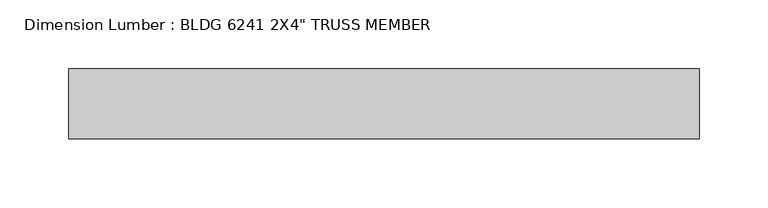
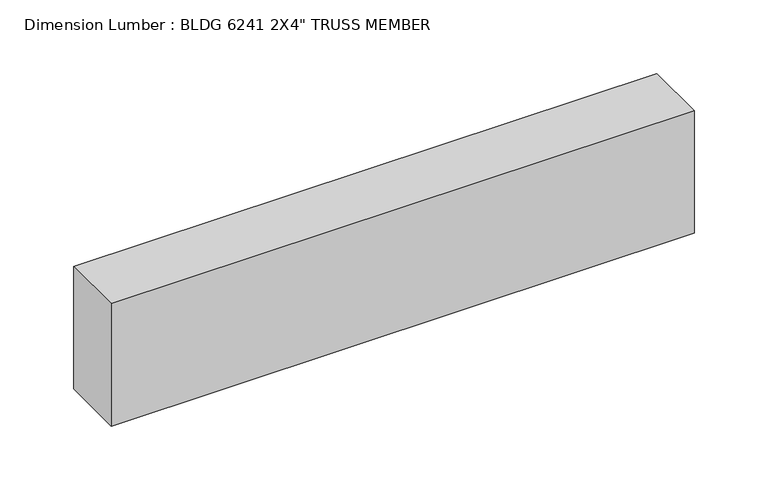
"""IFC4 building model written with IfcOpenShell, lengths in millimetres: beam geometry."""

from ifc_helpers import new_model, si_unit, frame, origin, place, context, project, spatial, polyline, outline, extrude, source, transform, mapped, element, save


def beam_154fe962(model_context):
    return source(origin(), model_context, "Body", "SweptSolid", [
        extrude(outline(polyline([(228.5999994, 25.4), (228.5999994, -25.4), (-228.6, -25.4), (-228.6, 25.4), (228.5999994, 25.4)])), frame((0.0, 0.0, -50.8), z_axis=(0.0, 0.0, 1.0), x_axis=(1.0, 0.0, 0.0)), (0.0, 0.0, 1.0), 101.6),
    ])


if __name__ == "__main__":
    model = new_model("IFC4")
    model_context = context("Model", 3, world=origin())
    ifc_project = project(units=[si_unit("LENGTHUNIT", "METRE", prefix="MILLI")], contexts=[model_context])
    site = spatial("IfcSite", under=ifc_project)
    building = spatial("IfcBuilding", under=site)
    placement = place(None, origin())
    beam_shape = beam_154fe962(model_context)
    element("IfcBeam", 1, ObjectType="Dimension Lumber : BLDG 6241 2X4\" TRUSS MEMBER", at=placement, inside=building, context=model_context, shape_type="MappedRepresentation", body=[
        mapped(beam_shape, transform((0.0, 0.0, 0.0), x_axis=(1.0, 0.0, 0.0), y_axis=(0.0, 1.0, 0.0), z_axis=(0.0, 0.0, 1.0))),
    ])
    save(model, "model.ifc")

# Revit data of these elements
# Type "Dimension Lumber : BLDG 6241 2X4\" TRUSS MEMBER"
#   Assembly Code = "B10"
#   A = 0.273472 SF
#   Length [instance default] = 5' - 0"
#   b = 0' - 2"
#   d = 0' - 4"
#   Structural Material [instance default] = Softwood, Lumber
# Element 1 (IfcBeam, "Dimension Lumber : BLDG 6241 2X4\" TRUSS MEMBER")
#   Materials on its faces: "Softwood, Lumber"
# Materials
#   "Softwood, Lumber": class "Wood", colour RGB 223 192 134, transparency 0, Description = "Pinus Echinata", Cost = 0
